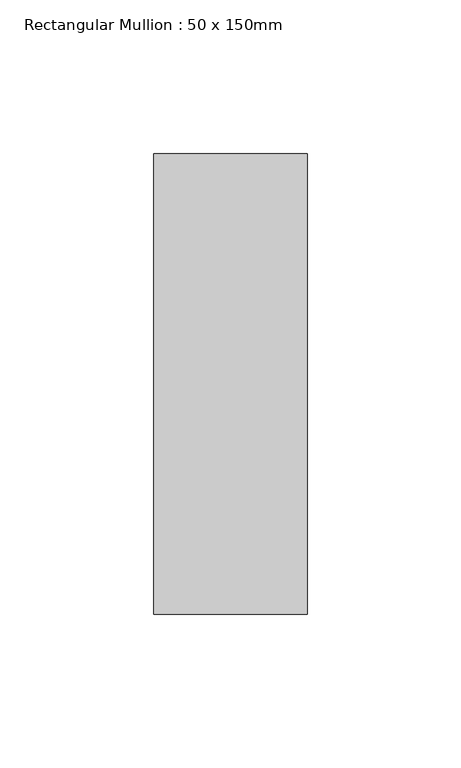
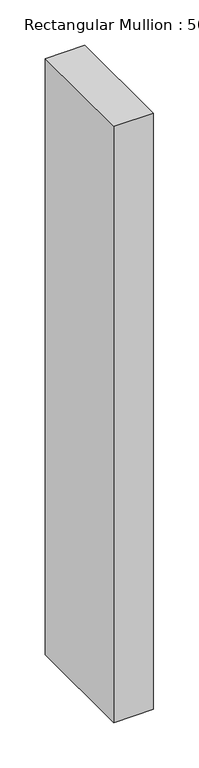
"""IFC4 building model written with IfcOpenShell, lengths in millimetres: member geometry, Rectangular Mullion : 50 x 150mm."""

import ifcopenshell
import ifcopenshell.guid

model = None  # the IFC model being written
_history = None  # IfcOwnerHistory: only IFC2X3 demands one
_inside = {}  # id of a spatial element -> (the spatial element, [elements in it])
_under = {}  # id of a project, library or spatial element -> (it, [spatial elements below it])
_declared = {}  # id of a project -> (the project, [libraries it declares])
_typed = {}  # id of a type object -> (the type object, [elements of that type])
_made_of = {}  # id of a material, layer set ... -> (it, [elements and type objects made of it])


def new_model(schema):
    """Start an empty IFC model of exactly this schema.

    Asked for "IFC4X3", IfcOpenShell would pick the latest addendum, in which some entities
    have other attributes; the version numbers below select the first issue.
    IFC2X3 requires an IfcOwnerHistory on every rooted entity: one is made here for all.
    """
    global model, _history
    if schema == "IFC4X3":
        model = ifcopenshell.file(schema_version=(4, 3, 0, 0))
    else:
        model = ifcopenshell.file(schema=schema)
    _inside.clear()
    _under.clear()
    _declared.clear()
    _typed.clear()
    _made_of.clear()
    _history = None
    if model.schema == "IFC2X3":
        org = make("IfcOrganization", Name="unknown")
        user = make(
            "IfcPersonAndOrganization",
            ThePerson=make("IfcPerson", FamilyName="unknown"),
            TheOrganization=org,
        )
        app = make(
            "IfcApplication",
            ApplicationDeveloper=org,
            Version="unknown",
            ApplicationFullName="unknown",
            ApplicationIdentifier="unknown",
        )
        _history = make(
            "IfcOwnerHistory",
            OwningUser=user,
            OwningApplication=app,
            ChangeAction="ADDED",
            CreationDate=0,
        )
    return model


def make(cls, **values):
    """One entity of the class cls with the attributes given. An attribute that is None is left unset."""
    return model.create_entity(
        cls, **{name: value for name, value in values.items() if value is not None}
    )


def rooted(cls, **values):
    """An entity with a GlobalId (a new one), such as an element, a storey or a relation."""
    return make(cls, GlobalId=ifcopenshell.guid.new(), OwnerHistory=_history, **values)


def si_unit(unit_type, name, prefix=None):
    """IfcSIUnit, for example si_unit("LENGTHUNIT", "METRE", prefix="MILLI")."""
    return make("IfcSIUnit", UnitType=unit_type, Prefix=prefix, Name=name)


def assignment(units):
    """IfcUnitAssignment: the units of a project."""
    return None if units is None else make("IfcUnitAssignment", Units=units)


def point(xyz):
    """IfcCartesianPoint."""
    return None if xyz is None else make("IfcCartesianPoint", Coordinates=xyz)


def direction(xyz):
    """IfcDirection."""
    return None if xyz is None else make("IfcDirection", DirectionRatios=xyz)


def frame(location, z_axis=None, x_axis=None):
    """IfcAxis2Placement3D, a coordinate frame: its origin and axes. An axis left out is left unset."""
    return make(
        "IfcAxis2Placement3D",
        Location=point(location),
        Axis=direction(z_axis),
        RefDirection=direction(x_axis),
    )


def origin():
    """The frame at (0, 0, 0) with its axes left unset."""
    return frame((0.0, 0.0, 0.0))


def place(relative_to, where):
    """IfcLocalPlacement: puts the frame where relative to a parent placement (None: the world)."""
    return make(
        "IfcLocalPlacement", PlacementRelTo=relative_to, RelativePlacement=where
    )


def context(
    kind, dimensions, precision=None, world=None, true_north=None, identifier=None
):
    """IfcGeometricRepresentationContext, for example the 3D "Model" context."""
    return make(
        "IfcGeometricRepresentationContext",
        ContextIdentifier=identifier,
        ContextType=kind,
        CoordinateSpaceDimension=dimensions,
        Precision=precision,
        WorldCoordinateSystem=world,
        TrueNorth=true_north,
    )


def project(units=None, contexts=None):
    """IfcProject with its units and contexts."""
    return rooted(
        "IfcProject",
        Name="project",
        RepresentationContexts=contexts,
        UnitsInContext=assignment(units),
    )


def spatial(cls, under=None, at=None, **own):
    """A site, building, storey or space (cls), placed at a placement, below another one or the project."""
    s = rooted(cls, ObjectPlacement=at, **own)
    if under is not None:
        _under.setdefault(under.id(), (under, []))[1].append(s)
    return s


def polyline(points):
    """IfcPolyline through the points."""
    return make("IfcPolyline", Points=[point(p) for p in points])


def outline(outer, holes=None, kind="AREA"):
    """IfcArbitraryClosedProfileDef: a profile drawn as a closed curve; with holes, ...WithVoids."""
    if holes is None:
        return make("IfcArbitraryClosedProfileDef", ProfileType=kind, OuterCurve=outer)
    return make(
        "IfcArbitraryProfileDefWithVoids",
        ProfileType=kind,
        OuterCurve=outer,
        InnerCurves=holes,
    )


def extrude(swept, where, along, depth):
    """IfcExtrudedAreaSolid: the profile swept, set in the frame where, extruded along a direction by depth."""
    return make(
        "IfcExtrudedAreaSolid",
        SweptArea=swept,
        Position=where,
        ExtrudedDirection=direction(along),
        Depth=depth,
    )


def shape(context_of_items, identifier, shape_type, items):
    """IfcShapeRepresentation: the items that make up one representation, for example the "Body"."""
    return make(
        "IfcShapeRepresentation",
        ContextOfItems=context_of_items,
        RepresentationIdentifier=identifier,
        RepresentationType=shape_type,
        Items=items,
    )


def source(mapping_origin, context_of_items, identifier, shape_type, items):
    """IfcRepresentationMap: a shape defined once, which mapped items show again and again."""
    return make(
        "IfcRepresentationMap",
        MappingOrigin=mapping_origin,
        MappedRepresentation=shape(context_of_items, identifier, shape_type, items),
    )


def transform(
    local_origin,
    x_axis=None,
    y_axis=None,
    z_axis=None,
    scale=None,
    scale2=None,
    scale3=None,
    uniform=True,
):
    """IfcCartesianTransformationOperator3D, or its non-uniform kind. x_axis, y_axis, z_axis: its Axis1, 2, 3."""
    if uniform:
        return make(
            "IfcCartesianTransformationOperator3D",
            Axis1=direction(x_axis),
            Axis2=direction(y_axis),
            LocalOrigin=point(local_origin),
            Scale=scale,
            Axis3=direction(z_axis),
        )
    return make(
        "IfcCartesianTransformationOperator3DnonUniform",
        Axis1=direction(x_axis),
        Axis2=direction(y_axis),
        LocalOrigin=point(local_origin),
        Scale=scale,
        Axis3=direction(z_axis),
        Scale2=scale2,
        Scale3=scale3,
    )


def mapped(mapping_source, mapping_target):
    """IfcMappedItem: shows the shape of a source again, moved by a transform."""
    return make(
        "IfcMappedItem", MappingSource=mapping_source, MappingTarget=mapping_target
    )


def made_of(thing, what):
    """Note that an element or type object is made of a material, layer set ...; save() writes the relation."""
    if what is not None:
        _made_of.setdefault(what.id(), (what, []))[1].append(thing)
    return thing


def element(
    cls,
    number,
    at=None,
    inside=None,
    cuts=None,
    type_object=None,
    material=None,
    context=None,
    identifier="Body",
    shape_type=None,
    held_by="IfcProductDefinitionShape",
    body=None,
    shapes=None,
    **own,
):
    """One element of the class cls, such as IfcWall. Its Tag is "e" and its number.

    at: its placement. inside: the storey or other place that contains it. cuts: it is an
    opening in that element (IfcRelVoidsElement). A single representation is given by context,
    identifier, shape_type and body (its items); several are given by shapes. held_by: the class
    of the entity that holds the representations. save() writes the other relations.
    """
    e = rooted(cls, Tag="e%d" % number, ObjectPlacement=at, **own)
    if body is not None:
        shapes = [shape(context, identifier, shape_type, body)]
    if shapes is not None:
        e.Representation = make(held_by, Representations=shapes)
    if inside is not None:
        _inside.setdefault(inside.id(), (inside, []))[1].append(e)
    if cuts is not None:
        rooted(
            "IfcRelVoidsElement", RelatingBuildingElement=cuts, RelatedOpeningElement=e
        )
    if type_object is not None:
        _typed.setdefault(type_object.id(), (type_object, []))[1].append(e)
    return made_of(e, material)


def aggregate(whole, parts):
    """IfcRelAggregates: a whole, such as a stair, and the parts it consists of."""
    return rooted("IfcRelAggregates", RelatingObject=whole, RelatedObjects=parts)


def save(model, path):
    """Write the relations noted so far, then the file.

    IfcRelAggregates (storeys below a building ...), IfcRelContainedInSpatialStructure (elements
    in a storey), IfcRelDefinesByType, IfcRelAssociatesMaterial and IfcRelDeclares: one each for
    every whole, place, type object, material and project.
    """
    for whole, parts in _under.values():
        aggregate(whole, parts)
    for where, things in _inside.values():
        rooted(
            "IfcRelContainedInSpatialStructure",
            RelatedElements=things,
            RelatingStructure=where,
        )
    for kind, things in _typed.values():
        rooted("IfcRelDefinesByType", RelatedObjects=things, RelatingType=kind)
    for what, things in _made_of.values():
        rooted("IfcRelAssociatesMaterial", RelatedObjects=things, RelatingMaterial=what)
    for by, libraries in _declared.values():
        rooted("IfcRelDeclares", RelatingContext=by, RelatedDefinitions=libraries)
    model.write(path)


def rectangular_mullion_50_x_150mm_6ffebc0f(model_context):
    return source(origin(), model_context, "Body", "SweptSolid", [
        extrude(outline(polyline([(0.0, 75.0), (0.0, -75.0), (-50.0, -75.0), (-50.0, 75.0), (0.0, 75.0)])), frame((0.0, 0.0, -800.0), z_axis=(0.0, 0.0, 1.0), x_axis=(1.0, 0.0, 0.0)), (0.0, 0.0, 1.0), 800.0),
    ])


if __name__ == "__main__":
    model = new_model("IFC4")
    model_context = context("Model", 3, world=origin())
    ifc_project = project(units=[si_unit("LENGTHUNIT", "METRE", prefix="MILLI")], contexts=[model_context])
    site = spatial("IfcSite", under=ifc_project)
    building = spatial("IfcBuilding", under=site)
    placement = place(None, origin())
    rectangular_mullion_50_x_150mm_shape = rectangular_mullion_50_x_150mm_6ffebc0f(model_context)
    element("IfcMember", 1, ObjectType="Rectangular Mullion : 50 x 150mm", at=placement, inside=building, context=model_context, shape_type="MappedRepresentation", body=[
        mapped(rectangular_mullion_50_x_150mm_shape, transform((0.0, 0.0, 0.0), x_axis=(1.0, 0.0, 0.0), y_axis=(0.0, 1.0, 0.0), z_axis=(0.0, 0.0, 1.0))),
    ])
    save(model, "model.ifc")

# Revit data of these elements
# Type "Rectangular Mullion : 50 x 150mm"
#   built-in parameter 1007304 = 0.492126 (stored number, unit not read)
#   built-in parameter 1007301 = 0.082021 (stored number, unit not read)
#   built-in parameter 1007300 = 0.082021 (stored number, unit not read)
# Element 1 (IfcMember, "Rectangular Mullion : 50 x 150mm")
#   Materials on its faces: "Metal - Aluminium"
# Materials
#   "Metal - Aluminium": class "Metal", colour RGB 247 247 247, transparency 0
